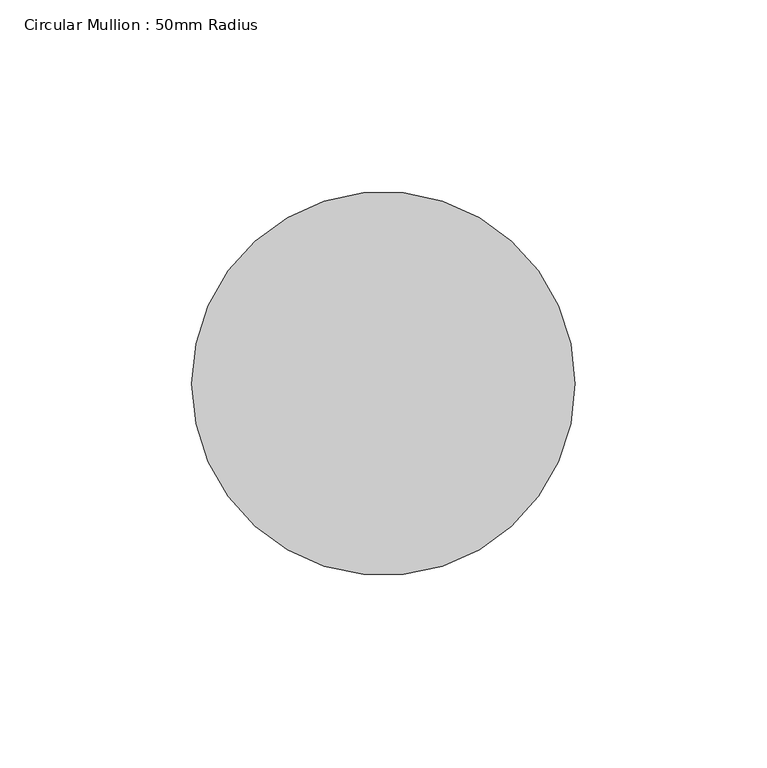
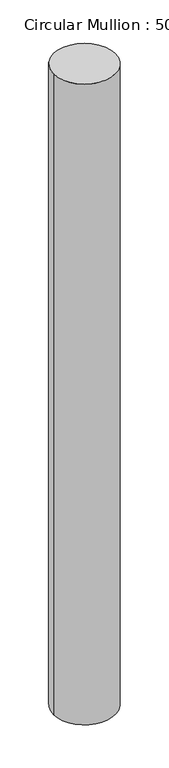
"""IFC4 building model written with IfcOpenShell, lengths in millimetres: member geometry, Circular Mullion : 50mm Radius."""

from ifc_helpers import new_model, si_unit, point, frame, origin, origin_2d, place, context, project, spatial, circle_curve, trimmed, segment, composite_curve, outline, extrude, source, transform, mapped, element, save


def circular_mullion_50mm_radius_3cb65144(model_context):
    return source(origin(), model_context, "Body", "SweptSolid", [
        extrude(outline(composite_curve([segment(trimmed(circle_curve(origin_2d(), 50.0), [point((50.0, 0.0))], [point((-50.0, 0.0))], False, "CARTESIAN"), True, "CONTINUOUS"), segment(trimmed(circle_curve(origin_2d(), 50.0), [point((-50.0, 0.0))], [point((50.0, 0.0))], False, "CARTESIAN"), True, "CONTINUOUS")], self_intersect=False)), frame((0.0, 0.0, -1094.2530538), z_axis=(0.0, 0.0, 1.0), x_axis=(1.0, 0.0, 0.0)), (0.0, 0.0, 1.0), 1094.2530538),
    ])


if __name__ == "__main__":
    model = new_model("IFC4")
    model_context = context("Model", 3, world=origin())
    ifc_project = project(units=[si_unit("LENGTHUNIT", "METRE", prefix="MILLI")], contexts=[model_context])
    site = spatial("IfcSite", under=ifc_project)
    building = spatial("IfcBuilding", under=site)
    placement = place(None, origin())
    circular_mullion_50mm_radius_shape = circular_mullion_50mm_radius_3cb65144(model_context)
    element("IfcMember", 1, ObjectType="Circular Mullion : 50mm Radius", at=placement, inside=building, context=model_context, shape_type="MappedRepresentation", body=[
        mapped(circular_mullion_50mm_radius_shape, transform((0.0, 0.0, 0.0), x_axis=(1.0, 0.0, 0.0), y_axis=(0.0, 1.0, 0.0), z_axis=(0.0, 0.0, 1.0))),
    ])
    save(model, "model.ifc")

# Revit data of these elements
# Type "Circular Mullion : 50mm Radius"
#   built-in parameter 1007350 = 0.164042 (stored number, unit not read)
# Element 1 (IfcMember, "Circular Mullion : 50mm Radius")
#   Materials on its faces: "Aluminium"
# Materials
#   "Aluminium": class "Metal", colour RGB 247 247 247, transparency 0, Description = "Aluminium 6061", Cost = 0
